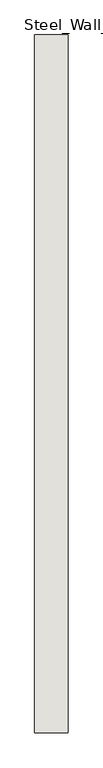
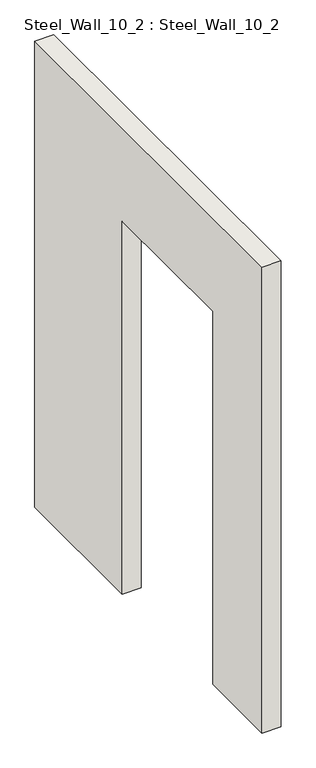
"""IFC4 building model written with IfcOpenShell, lengths in millimetres: wall geometry, Steel_Wall_10_2 : Steel_Wall_10_2."""

from ifc_helpers import new_model, si_unit, frame, origin, place, context, project, spatial, polyline, outline, extrude, source, transform, mapped, element, save


def steel_wall_10_2_steel_wall_10_2_ac5a625b(model_context):
    return source(origin(), model_context, "Body", "SweptSolid", [
        extrude(outline(polyline([(7515.0, 2850.0), (9595.0, 2850.0), (9595.0, 250.0), (8795.0, 250.0), (8795.0, 2330.0), (7965.0, 2330.0), (7965.0, 250.0), (7515.0, 250.0), (7515.0, 2850.0)])), frame((4265.0, 0.0, 0.0), z_axis=(1.0, 0.0, 0.0), x_axis=(0.0, 1.0, 0.0)), (0.0, 0.0, 1.0), 100.0),
    ])


if __name__ == "__main__":
    model = new_model("IFC4")
    model_context = context("Model", 3, world=origin())
    ifc_project = project(units=[si_unit("LENGTHUNIT", "METRE", prefix="MILLI")], contexts=[model_context])
    site = spatial("IfcSite", under=ifc_project)
    building = spatial("IfcBuilding", under=site)
    placement = place(None, origin())
    steel_wall_10_2_steel_wall_10_2_shape = steel_wall_10_2_steel_wall_10_2_ac5a625b(model_context)
    element("IfcWall", 1, ObjectType="Steel_Wall_10_2 : Steel_Wall_10_2", at=placement, inside=building, context=model_context, shape_type="MappedRepresentation", body=[
        mapped(steel_wall_10_2_steel_wall_10_2_shape, transform((0.0, 0.0, 0.0), x_axis=(1.0, 0.0, 0.0), y_axis=(0.0, 1.0, 0.0), z_axis=(0.0, 0.0, 1.0))),
    ])
    save(model, "model.ifc")

# Revit data of these elements
# Type "Steel_Wall_10_2 : Steel_Wall_10_2"
#   NameOverride = "Steel_Wall_10_2"
# Element 1 (IfcWall, "Steel_Wall_10_2 : Steel_Wall_10_2")
#   Materials on its faces: "IfcSurfaceStyle #33"
# Materials
#   "IfcSurfaceStyle #33": class "Unassigned", colour RGB 214 214 214, transparency 0
